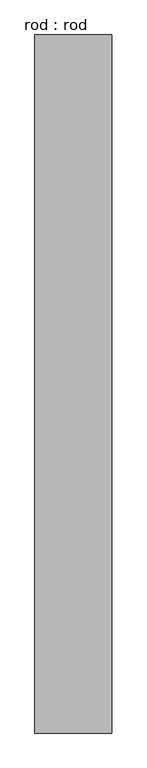
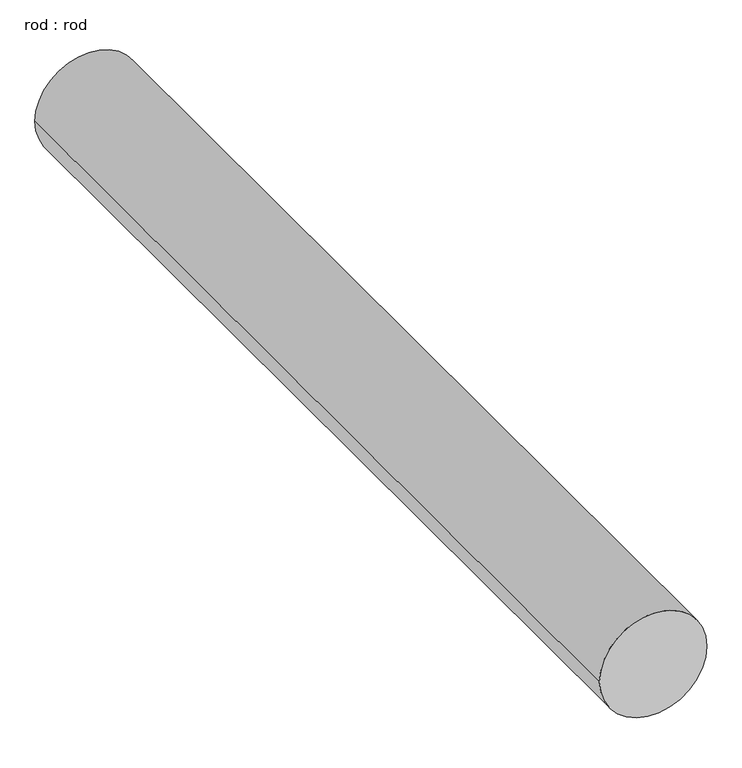
"""IFC4 building model written with IfcOpenShell, lengths in millimetres: proxy geometry, rod : rod."""

from ifc_helpers import new_model, si_unit, point, frame, frame_2d, origin, place, context, project, spatial, circle_curve, trimmed, segment, composite_curve, outline, extrude, source, transform, mapped, element, save


def rod_rod_dcd340a7(model_context):
    return source(origin(), model_context, "Body", "SweptSolid", [
        extrude(outline(composite_curve([segment(trimmed(circle_curve(frame_2d((0.0108462, 0.0)), 200.0), [point((0.0108462, 200.0))], [point((0.0108462, -200.0))], False, "CARTESIAN"), True, "CONTINUOUS"), segment(trimmed(circle_curve(frame_2d((0.0108462, 0.0)), 200.0), [point((0.0108462, -200.0))], [point((0.0108462, 200.0))], False, "CARTESIAN"), True, "CONTINUOUS")], self_intersect=False)), frame((0.0, 2273.729921, 0.0), z_axis=(0.0, 1.0, 0.0), x_axis=(0.0, 0.0, 1.0)), (0.0, 0.0, 1.0), 3637.9973887),
    ])


if __name__ == "__main__":
    model = new_model("IFC4")
    model_context = context("Model", 3, world=origin())
    ifc_project = project(units=[si_unit("LENGTHUNIT", "METRE", prefix="MILLI")], contexts=[model_context])
    site = spatial("IfcSite", under=ifc_project)
    building = spatial("IfcBuilding", under=site)
    placement = place(None, origin())
    rod_rod_shape = rod_rod_dcd340a7(model_context)
    element("IfcBuildingElementProxy", 1, Name="rod : rod", ObjectType="rod : rod", at=placement, inside=building, context=model_context, shape_type="MappedRepresentation", body=[
        mapped(rod_rod_shape, transform((0.0, 0.0, 0.0), x_axis=(1.0, 0.0, 0.0), y_axis=(0.0, 1.0, 0.0), z_axis=(0.0, 0.0, 1.0))),
    ])
    save(model, "model.ifc")

# Revit data of these elements
# Type "rod : rod"
#   Default Elevation = 0
